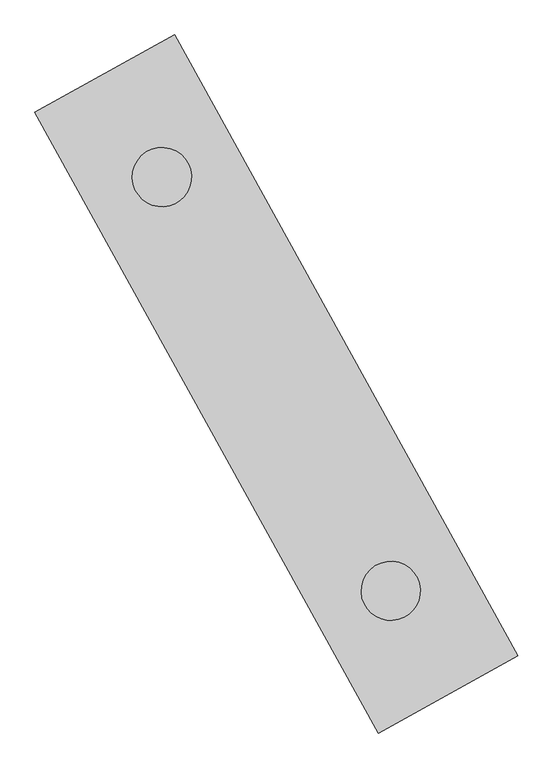
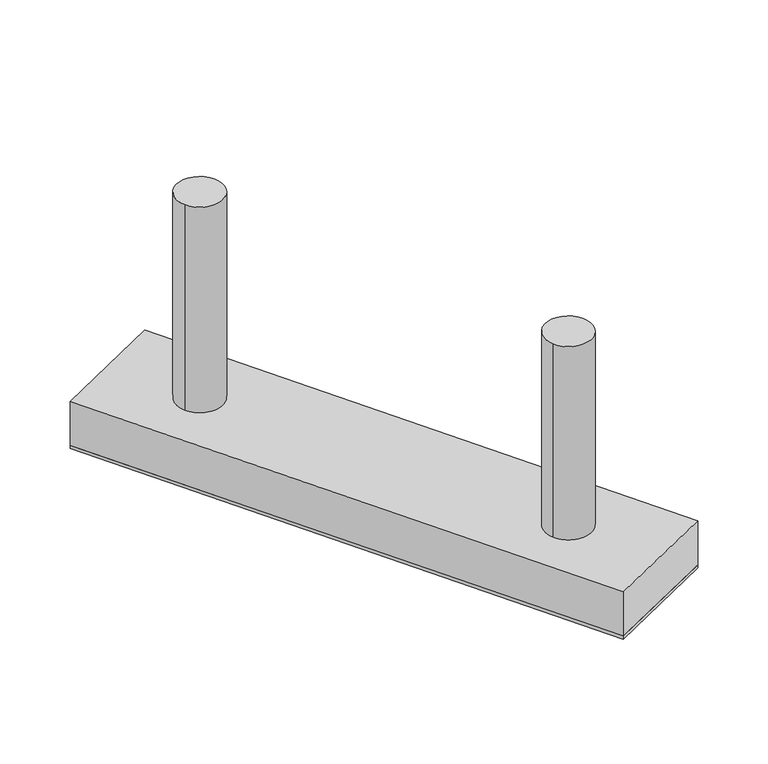
"""IFC4 building model written with IfcOpenShell, lengths in millimetres: beam geometry, KNA_SF_TSP as2 : KNA_SF_TSP as2."""

import ifcopenshell
import ifcopenshell.guid

model = None  # the IFC model being written
_history = None  # IfcOwnerHistory: only IFC2X3 demands one
_inside = {}  # id of a spatial element -> (the spatial element, [elements in it])
_under = {}  # id of a project, library or spatial element -> (it, [spatial elements below it])
_declared = {}  # id of a project -> (the project, [libraries it declares])
_typed = {}  # id of a type object -> (the type object, [elements of that type])
_made_of = {}  # id of a material, layer set ... -> (it, [elements and type objects made of it])


def new_model(schema):
    """Start an empty IFC model of exactly this schema.

    Asked for "IFC4X3", IfcOpenShell would pick the latest addendum, in which some entities
    have other attributes; the version numbers below select the first issue.
    IFC2X3 requires an IfcOwnerHistory on every rooted entity: one is made here for all.
    """
    global model, _history
    if schema == "IFC4X3":
        model = ifcopenshell.file(schema_version=(4, 3, 0, 0))
    else:
        model = ifcopenshell.file(schema=schema)
    _inside.clear()
    _under.clear()
    _declared.clear()
    _typed.clear()
    _made_of.clear()
    _history = None
    if model.schema == "IFC2X3":
        org = make("IfcOrganization", Name="unknown")
        user = make(
            "IfcPersonAndOrganization",
            ThePerson=make("IfcPerson", FamilyName="unknown"),
            TheOrganization=org,
        )
        app = make(
            "IfcApplication",
            ApplicationDeveloper=org,
            Version="unknown",
            ApplicationFullName="unknown",
            ApplicationIdentifier="unknown",
        )
        _history = make(
            "IfcOwnerHistory",
            OwningUser=user,
            OwningApplication=app,
            ChangeAction="ADDED",
            CreationDate=0,
        )
    return model


def make(cls, **values):
    """One entity of the class cls with the attributes given. An attribute that is None is left unset."""
    return model.create_entity(
        cls, **{name: value for name, value in values.items() if value is not None}
    )


def rooted(cls, **values):
    """An entity with a GlobalId (a new one), such as an element, a storey or a relation."""
    return make(cls, GlobalId=ifcopenshell.guid.new(), OwnerHistory=_history, **values)


def si_unit(unit_type, name, prefix=None):
    """IfcSIUnit, for example si_unit("LENGTHUNIT", "METRE", prefix="MILLI")."""
    return make("IfcSIUnit", UnitType=unit_type, Prefix=prefix, Name=name)


def assignment(units):
    """IfcUnitAssignment: the units of a project."""
    return None if units is None else make("IfcUnitAssignment", Units=units)


def point(xyz):
    """IfcCartesianPoint."""
    return None if xyz is None else make("IfcCartesianPoint", Coordinates=xyz)


def direction(xyz):
    """IfcDirection."""
    return None if xyz is None else make("IfcDirection", DirectionRatios=xyz)


def frame(location, z_axis=None, x_axis=None):
    """IfcAxis2Placement3D, a coordinate frame: its origin and axes. An axis left out is left unset."""
    return make(
        "IfcAxis2Placement3D",
        Location=point(location),
        Axis=direction(z_axis),
        RefDirection=direction(x_axis),
    )


def frame_2d(location, x_axis=None):
    """IfcAxis2Placement2D, a coordinate frame in the plane: its origin and x axis."""
    return make(
        "IfcAxis2Placement2D", Location=point(location), RefDirection=direction(x_axis)
    )


def origin():
    """The frame at (0, 0, 0) with its axes left unset."""
    return frame((0.0, 0.0, 0.0))


def place(relative_to, where):
    """IfcLocalPlacement: puts the frame where relative to a parent placement (None: the world)."""
    return make(
        "IfcLocalPlacement", PlacementRelTo=relative_to, RelativePlacement=where
    )


def context(
    kind, dimensions, precision=None, world=None, true_north=None, identifier=None
):
    """IfcGeometricRepresentationContext, for example the 3D "Model" context."""
    return make(
        "IfcGeometricRepresentationContext",
        ContextIdentifier=identifier,
        ContextType=kind,
        CoordinateSpaceDimension=dimensions,
        Precision=precision,
        WorldCoordinateSystem=world,
        TrueNorth=true_north,
    )


def project(units=None, contexts=None):
    """IfcProject with its units and contexts."""
    return rooted(
        "IfcProject",
        Name="project",
        RepresentationContexts=contexts,
        UnitsInContext=assignment(units),
    )


def spatial(cls, under=None, at=None, **own):
    """A site, building, storey or space (cls), placed at a placement, below another one or the project."""
    s = rooted(cls, ObjectPlacement=at, **own)
    if under is not None:
        _under.setdefault(under.id(), (under, []))[1].append(s)
    return s


def polyline(points):
    """IfcPolyline through the points."""
    return make("IfcPolyline", Points=[point(p) for p in points])


def circle_curve(where, radius):
    """IfcCircle in the frame where."""
    return make("IfcCircle", Position=where, Radius=radius)


def trimmed(basis, trim1, trim2, sense, master):
    """IfcTrimmedCurve: the piece of a basis curve between two trims."""
    return make(
        "IfcTrimmedCurve",
        BasisCurve=basis,
        Trim1=trim1,
        Trim2=trim2,
        SenseAgreement=sense,
        MasterRepresentation=master,
    )


def segment(curve, same_sense, transition):
    """IfcCompositeCurveSegment."""
    return make(
        "IfcCompositeCurveSegment",
        Transition=transition,
        SameSense=same_sense,
        ParentCurve=curve,
    )


def composite_curve(segments, self_intersect=None):
    """IfcCompositeCurve: segments joined end to end."""
    return make("IfcCompositeCurve", Segments=segments, SelfIntersect=self_intersect)


def outline(outer, holes=None, kind="AREA"):
    """IfcArbitraryClosedProfileDef: a profile drawn as a closed curve; with holes, ...WithVoids."""
    if holes is None:
        return make("IfcArbitraryClosedProfileDef", ProfileType=kind, OuterCurve=outer)
    return make(
        "IfcArbitraryProfileDefWithVoids",
        ProfileType=kind,
        OuterCurve=outer,
        InnerCurves=holes,
    )


def extrude(swept, where, along, depth):
    """IfcExtrudedAreaSolid: the profile swept, set in the frame where, extruded along a direction by depth."""
    return make(
        "IfcExtrudedAreaSolid",
        SweptArea=swept,
        Position=where,
        ExtrudedDirection=direction(along),
        Depth=depth,
    )


def shape(context_of_items, identifier, shape_type, items):
    """IfcShapeRepresentation: the items that make up one representation, for example the "Body"."""
    return make(
        "IfcShapeRepresentation",
        ContextOfItems=context_of_items,
        RepresentationIdentifier=identifier,
        RepresentationType=shape_type,
        Items=items,
    )


def source(mapping_origin, context_of_items, identifier, shape_type, items):
    """IfcRepresentationMap: a shape defined once, which mapped items show again and again."""
    return make(
        "IfcRepresentationMap",
        MappingOrigin=mapping_origin,
        MappedRepresentation=shape(context_of_items, identifier, shape_type, items),
    )


def transform(
    local_origin,
    x_axis=None,
    y_axis=None,
    z_axis=None,
    scale=None,
    scale2=None,
    scale3=None,
    uniform=True,
):
    """IfcCartesianTransformationOperator3D, or its non-uniform kind. x_axis, y_axis, z_axis: its Axis1, 2, 3."""
    if uniform:
        return make(
            "IfcCartesianTransformationOperator3D",
            Axis1=direction(x_axis),
            Axis2=direction(y_axis),
            LocalOrigin=point(local_origin),
            Scale=scale,
            Axis3=direction(z_axis),
        )
    return make(
        "IfcCartesianTransformationOperator3DnonUniform",
        Axis1=direction(x_axis),
        Axis2=direction(y_axis),
        LocalOrigin=point(local_origin),
        Scale=scale,
        Axis3=direction(z_axis),
        Scale2=scale2,
        Scale3=scale3,
    )


def mapped(mapping_source, mapping_target):
    """IfcMappedItem: shows the shape of a source again, moved by a transform."""
    return make(
        "IfcMappedItem", MappingSource=mapping_source, MappingTarget=mapping_target
    )


def made_of(thing, what):
    """Note that an element or type object is made of a material, layer set ...; save() writes the relation."""
    if what is not None:
        _made_of.setdefault(what.id(), (what, []))[1].append(thing)
    return thing


def element(
    cls,
    number,
    at=None,
    inside=None,
    cuts=None,
    type_object=None,
    material=None,
    context=None,
    identifier="Body",
    shape_type=None,
    held_by="IfcProductDefinitionShape",
    body=None,
    shapes=None,
    **own,
):
    """One element of the class cls, such as IfcWall. Its Tag is "e" and its number.

    at: its placement. inside: the storey or other place that contains it. cuts: it is an
    opening in that element (IfcRelVoidsElement). A single representation is given by context,
    identifier, shape_type and body (its items); several are given by shapes. held_by: the class
    of the entity that holds the representations. save() writes the other relations.
    """
    e = rooted(cls, Tag="e%d" % number, ObjectPlacement=at, **own)
    if body is not None:
        shapes = [shape(context, identifier, shape_type, body)]
    if shapes is not None:
        e.Representation = make(held_by, Representations=shapes)
    if inside is not None:
        _inside.setdefault(inside.id(), (inside, []))[1].append(e)
    if cuts is not None:
        rooted(
            "IfcRelVoidsElement", RelatingBuildingElement=cuts, RelatedOpeningElement=e
        )
    if type_object is not None:
        _typed.setdefault(type_object.id(), (type_object, []))[1].append(e)
    return made_of(e, material)


def aggregate(whole, parts):
    """IfcRelAggregates: a whole, such as a stair, and the parts it consists of."""
    return rooted("IfcRelAggregates", RelatingObject=whole, RelatedObjects=parts)


def save(model, path):
    """Write the relations noted so far, then the file.

    IfcRelAggregates (storeys below a building ...), IfcRelContainedInSpatialStructure (elements
    in a storey), IfcRelDefinesByType, IfcRelAssociatesMaterial and IfcRelDeclares: one each for
    every whole, place, type object, material and project.
    """
    for whole, parts in _under.values():
        aggregate(whole, parts)
    for where, things in _inside.values():
        rooted(
            "IfcRelContainedInSpatialStructure",
            RelatedElements=things,
            RelatingStructure=where,
        )
    for kind, things in _typed.values():
        rooted("IfcRelDefinesByType", RelatedObjects=things, RelatingType=kind)
    for what, things in _made_of.values():
        rooted("IfcRelAssociatesMaterial", RelatedObjects=things, RelatingMaterial=what)
    for by, libraries in _declared.values():
        rooted("IfcRelDeclares", RelatingContext=by, RelatedDefinitions=libraries)
    model.write(path)


def beam_c9faa05f(model_context):
    return source(origin(), model_context, "Body", "SweptSolid", [
        extrude(outline(composite_curve([segment(trimmed(circle_curve(frame_2d((135664.8983796, -46523.8745389)), 500.0), [point((135215.6906298, -46743.4477557))], [point((136114.1061294, -46304.3013221))], False, "CARTESIAN"), True, "CONTINUOUS"), segment(trimmed(circle_curve(frame_2d((135664.8983796, -46523.8745389)), 500.0), [point((136114.1061294, -46304.3013221))], [point((135215.6906298, -46743.4477557))], False, "CARTESIAN"), True, "CONTINUOUS")], self_intersect=False)), frame((0.0, 0.0, -1600.0), z_axis=(0.0, 0.0, 1.0), x_axis=(1.0, 0.0, 0.0)), (0.0, 0.0, 1.0), 4389.7791108),
        extrude(outline(composite_curve([segment(trimmed(circle_curve(frame_2d((131790.1548192, -39524.8487252)), 500.0), [point((131340.9470694, -39744.421942))], [point((132239.3625689, -39305.2755084))], False, "CARTESIAN"), True, "CONTINUOUS"), segment(trimmed(circle_curve(frame_2d((131790.1548192, -39524.8487252)), 500.0), [point((132239.3625689, -39305.2755084))], [point((131340.9470694, -39744.421942))], False, "CARTESIAN"), True, "CONTINUOUS")], self_intersect=False)), frame((0.0, 0.0, -1600.0), z_axis=(0.0, 0.0, 1.0), x_axis=(1.0, 0.0, 0.0)), (0.0, 0.0, 1.0), 4669.040393),
        extrude(outline(polyline([(129640.383323, -38428.9552476), (132002.5545351, -37121.2292959), (137814.6698758, -47619.7680165), (135452.4986636, -48927.4939681), (129640.383323, -38428.9552476)])), frame((0.0, 0.0, -2600.0), z_axis=(0.0, 0.0, 1.0), x_axis=(1.0, 0.0, 0.0)), (0.0, 0.0, 1.0), 1000.0),
        extrude(outline(polyline([(129640.383323, -38428.9552476), (132002.5545351, -37121.2292959), (137814.6698758, -47619.7680165), (135452.4986636, -48927.4939681), (129640.383323, -38428.9552476)])), frame((0.0, 0.0, -2670.0), z_axis=(0.0, 0.0, 1.0), x_axis=(1.0, 0.0, 0.0)), (0.0, 0.0, 1.0), 70.0),
    ])


if __name__ == "__main__":
    model = new_model("IFC4")
    model_context = context("Model", 3, world=origin())
    ifc_project = project(units=[si_unit("LENGTHUNIT", "METRE", prefix="MILLI")], contexts=[model_context])
    site = spatial("IfcSite", under=ifc_project)
    building = spatial("IfcBuilding", under=site)
    placement = place(None, origin())
    beam_shape = beam_c9faa05f(model_context)
    element("IfcBeam", 1, ObjectType="KNA_SF_TSP as2 : KNA_SF_TSP as2", at=placement, inside=building, context=model_context, shape_type="MappedRepresentation", body=[
        mapped(beam_shape, transform((0.0, 0.0, 0.0), x_axis=(1.0, 0.0, 0.0), y_axis=(0.0, 1.0, 0.0), z_axis=(0.0, 0.0, 1.0))),
    ])
    save(model, "model.ifc")

# Revit data of these elements
# Element 1 (IfcBeam, "KNA_SF_TSP as2 : KNA_SF_TSP as2")
#   Materials on its faces: "Beton_Bestaande Constructie", "Beton_In-Situ_Werkvloer"
# Materials
#   "Beton_Bestaande Constructie": class "Concrete", colour RGB 102 102 102, transparency 0, Description = "Beton", Cost = 0
#   "Beton_In-Situ_Werkvloer": class "Concrete", colour RGB 128 128 128, transparency 0, Description = "Beton", Cost = 0
